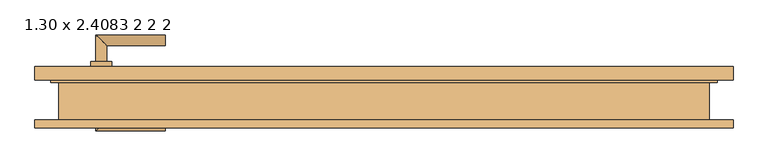
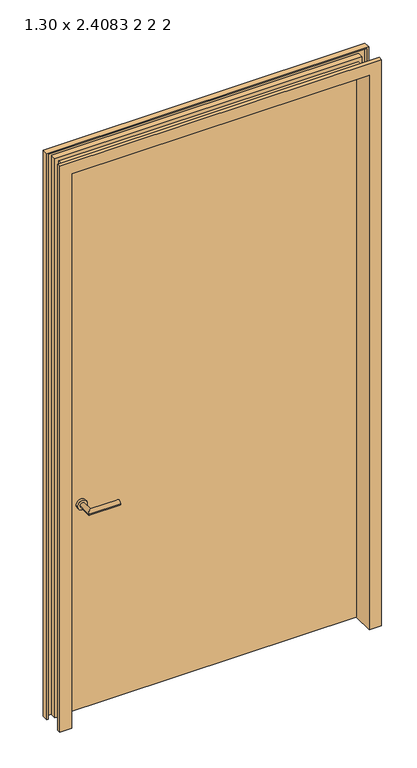
"""IFC4 building model written with IfcOpenShell, lengths in millimetres: door geometry, Drehflügel 1-flg - Stahlzarge : 1.30 x 2.4083 2 2 2."""

from ifc_helpers import new_model, si_unit, point, frame, frame_2d, origin, place, context, project, spatial, polyline, circle_curve, ellipse_curve, trimmed, segment, composite_curve, outline, extrude, faceted_brep, source, transform, mapped, element, save
from ifc_brep_helpers import plane_surface, cylinder_surface, advanced_brep


def door_1_30_x_2_4083_2_2_2_2f50041d(model_context):
    return source(origin(), model_context, "Body", "SolidModel", [
        advanced_brep(
        [(-540.0, 26.9346141, 915.0), (-520.0, 26.9346141, 915.0), (-540.0, -43.0653859, 915.0), (-520.0, -23.0653859, 915.0), (-410.0, -43.0653859, 915.0), (-410.0, -23.0653859, 915.0)],
        [
            (0, 1, circle_curve(frame((-530.0, 26.9346141, 915.0), z_axis=(0.0, 1.0, 0.0), x_axis=(1.0, 0.0, 0.0)), 10.0)),
            (1, 0, circle_curve(frame((-530.0, 26.9346141, 915.0), z_axis=(0.0, 1.0, 0.0), x_axis=(1.0, 0.0, 0.0)), 10.0)),
            (0, 2),
            (2, 3, ellipse_curve(frame((-530.0, -33.0653859, 915.0), z_axis=(-0.7071067811865385, 0.7071067811865565, 0.0), x_axis=(0.7071067811865563, 0.7071067811865386, 0.0)), 14.1421356, 10.0)),
            (3, 1),
            (3, 2, ellipse_curve(frame((-530.0, -33.0653859, 915.0), z_axis=(-0.7071067811865385, 0.7071067811865565, 0.0), x_axis=(0.7071067811865563, 0.7071067811865386, 0.0)), 14.1421356, 10.0)),
            (4, 5, circle_curve(frame((-410.0, -33.0653859, 915.0), z_axis=(1.0, 0.0, 0.0), x_axis=(0.0, 1.0, 0.0)), 10.0)),
            (5, 4, circle_curve(frame((-410.0, -33.0653859, 915.0), z_axis=(1.0, 0.0, 0.0), x_axis=(0.0, 1.0, 0.0)), 10.0)),
            (2, 4),
            (5, 3),
        ],
        [
            plane_surface(frame((-530.0, 26.9346141, -372.7526403), z_axis=(0.0, 1.0, 0.0), x_axis=(0.0, 0.0, 1.0))),
            cylinder_surface(frame((-530.0, 26.9346141, 915.0), z_axis=(0.0, 1.0, 0.0), x_axis=(1.0, 0.0, 0.0)), 10.0),
            plane_surface(frame((-410.0, -33.0653859, -372.7526403), z_axis=(1.0, 0.0, 0.0), x_axis=(0.0, 0.0, 1.0))),
            cylinder_surface(frame((-530.0, -33.0653859, 915.0), z_axis=(-1.0, 0.0, 0.0), x_axis=(0.0, 1.0, 0.0)), 10.0),
        ],
        [
            (0, [[1, 2]]),
            (1, [[-1, 3, 4, 5]]),
            (1, [[-2, -5, 6, -3]]),
            (2, [[7, 8]]),
            (3, [[-4, 9, -8, 10]]),
            (3, [[-6, -10, -7, -9]]),
        ],
    ),
        advanced_brep(
        [(-520.0, 86.9346141, 915.0), (-540.0, 86.9346141, 915.0), (-520.0, 116.9346141, 915.0), (-540.0, 136.9346141, 915.0), (-410.0, 116.9346141, 915.0), (-410.0, 136.9346141, 915.0)],
        [
            (0, 1, circle_curve(frame((-530.0, 86.9346141, 915.0), z_axis=(0.0, -1.0, 0.0), x_axis=(-1.0, 0.0, 0.0)), 10.0)),
            (1, 0, circle_curve(frame((-530.0, 86.9346141, 915.0), z_axis=(0.0, -1.0, 0.0), x_axis=(-1.0, 0.0, 0.0)), 10.0)),
            (0, 2),
            (2, 3, ellipse_curve(frame((-530.0, 126.9346141, 915.0), z_axis=(-0.7071067811865475, -0.7071067811865475, 0.0), x_axis=(0.7071067811865474, -0.7071067811865476, 0.0)), 14.1421356, 10.0)),
            (3, 1),
            (3, 2, ellipse_curve(frame((-530.0, 126.9346141, 915.0), z_axis=(-0.7071067811865475, -0.7071067811865475, 0.0), x_axis=(0.7071067811865474, -0.7071067811865476, 0.0)), 14.1421356, 10.0)),
            (4, 5, circle_curve(frame((-410.0, 126.9346141, 915.0), z_axis=(1.0, 0.0, 0.0), x_axis=(0.0, 1.0, 0.0)), 10.0)),
            (5, 4, circle_curve(frame((-410.0, 126.9346141, 915.0), z_axis=(1.0, 0.0, 0.0), x_axis=(0.0, 1.0, 0.0)), 10.0)),
            (2, 4),
            (5, 3),
        ],
        [
            plane_surface(frame((-530.0, 86.9346141, -372.7526403), z_axis=(0.0, -1.0, 0.0), x_axis=(0.0, 0.0, 1.0))),
            cylinder_surface(frame((-530.0, 86.9346141, 915.0), z_axis=(0.0, -1.0, 0.0), x_axis=(-1.0, 0.0, 0.0)), 10.0),
            plane_surface(frame((-410.0, 126.9346141, -372.7526403), z_axis=(1.0, 0.0, 0.0), x_axis=(0.0, 0.0, 1.0))),
            cylinder_surface(frame((-530.0, 126.9346141, 915.0), z_axis=(-1.0, 0.0, 0.0), x_axis=(0.0, 1.0, 0.0)), 10.0),
        ],
        [
            (0, [[1, 2]]),
            (1, [[-1, 3, 4, 5]]),
            (1, [[-2, -5, 6, -3]]),
            (2, [[7, 8]]),
            (3, [[-4, 9, -8, 10]]),
            (3, [[-6, -10, -7, -9]]),
        ],
    ),
        extrude(outline(composite_curve([segment(trimmed(circle_curve(frame_2d((915.0, -530.0)), 20.0), [point((915.0, -550.0))], [point((915.0, -510.0))], False, "CARTESIAN"), True, "CONTINUOUS"), segment(trimmed(circle_curve(frame_2d((915.0, -530.0)), 20.0), [point((915.0, -510.0))], [point((915.0, -550.0))], False, "CARTESIAN"), True, "CONTINUOUS")], self_intersect=False)), frame((0.0, 16.9346141, 0.0), z_axis=(0.0, 1.0, 0.0), x_axis=(0.0, 0.0, 1.0)), (0.0, 0.0, 1.0), 10.0),
        extrude(outline(composite_curve([segment(trimmed(circle_curve(frame_2d((915.0, -530.0)), 20.0), [point((915.0, -550.0))], [point((915.0, -510.0))], False, "CARTESIAN"), True, "CONTINUOUS"), segment(trimmed(circle_curve(frame_2d((915.0, -530.0)), 20.0), [point((915.0, -510.0))], [point((915.0, -550.0))], False, "CARTESIAN"), True, "CONTINUOUS")], self_intersect=False)), frame((0.0, 76.9346141, 0.0), z_axis=(0.0, 1.0, 0.0), x_axis=(0.0, 0.0, 1.0)), (0.0, 0.0, 1.0), 10.0),
        extrude(outline(polyline([(620.0, 51.9346141), (-620.0, 51.9346141), (-620.0, 76.9346141), (620.0, 76.9346141), (620.0, 51.9346141)])), frame((0.0, 0.0, 15.0), z_axis=(0.0, 0.0, 1.0), x_axis=(1.0, 0.0, 0.0)), (0.0, 0.0, 1.0), 2398.3),
        faceted_brep([(654.4603207, -38.0653859, 15.0), (605.0, -38.0653859, 15.0), (605.0, 51.9346141, 15.0), (620.0, 51.9346141, 15.0), (620.0, 76.9346141, 15.0), (654.4603207, 76.9346141, 15.0), (654.4603207, 51.9346141, 15.0), (649.4603207, 51.9346141, 15.0), (649.4603207, 71.9346141, 15.0), (625.0, 71.9346141, 15.0), (625.0, 46.9346141, 15.0), (610.0, 46.9346141, 15.0), (610.0, -33.0653859, 15.0), (649.4603207, -33.0653859, 15.0), (649.4603207, -23.0653859, 15.0), (654.4603207, -23.0653859, 15.0), (654.4603207, -38.0653859, 2447.7603207), (-654.4603207, -38.0653859, 2447.7603207), (-654.4603207, -38.0653859, 15.0), (-605.0, -38.0653859, 15.0), (-605.0, -38.0653859, 2398.3), (605.0, -38.0653859, 2398.3), (605.0, 51.9346141, 2398.3), (-605.0, 51.9346141, 2398.3), (-605.0, 51.9346141, 15.0), (-620.0, 51.9346141, 15.0), (-620.0, 51.9346141, 2413.3), (620.0, 51.9346141, 2413.3), (620.0, 76.9346141, 2413.3), (-620.0, 76.9346141, 2413.3), (-620.0, 76.9346141, 15.0), (-654.4603207, 76.9346141, 15.0), (-654.4603207, 76.9346141, 2447.7603207), (654.4603207, 76.9346141, 2447.7603207), (654.4603207, 51.9346141, 2447.7603207), (-654.4603207, 51.9346141, 2447.7603207), (-654.4603207, 51.9346141, 15.0), (-649.4603207, 51.9346141, 15.0), (-649.4603207, 51.9346141, 2442.7603207), (649.4603207, 51.9346141, 2442.7603207), (649.4603207, 71.9346141, 2442.7603207), (-649.4603207, 71.9346141, 2442.7603207), (-649.4603207, 71.9346141, 15.0), (-625.0, 71.9346141, 15.0), (-625.0, 71.9346141, 2418.3), (625.0, 71.9346141, 2418.3), (625.0, 46.9346141, 2418.3), (-625.0, 46.9346141, 2418.3), (-625.0, 46.9346141, 15.0), (-610.0, 46.9346141, 15.0), (-610.0, 46.9346141, 2403.3), (610.0, 46.9346141, 2403.3), (610.0, -33.0653859, 2403.3), (-610.0, -33.0653859, 2403.3), (-610.0, -33.0653859, 15.0), (-649.4603207, -33.0653859, 15.0), (-649.4603207, -33.0653859, 2442.7603207), (649.4603207, -33.0653859, 2442.7603207), (649.4603207, -23.0653859, 2442.7603207), (-649.4603207, -23.0653859, 2442.7603207), (-649.4603207, -23.0653859, 15.0), (-654.4603207, -23.0653859, 15.0), (-654.4603207, -23.0653859, 2447.7603207), (654.4603207, -23.0653859, 2447.7603207)], [[[0, 1, 2, 3, 4, 5, 6, 7, 8, 9, 10, 11, 12, 13, 14, 15]], [[1, 0, 16, 17, 18, 19, 20, 21]], [[2, 1, 21, 22]], [[3, 2, 22, 23, 24, 25, 26, 27]], [[4, 3, 27, 28]], [[5, 4, 28, 29, 30, 31, 32, 33]], [[6, 5, 33, 34]], [[7, 6, 34, 35, 36, 37, 38, 39]], [[8, 7, 39, 40]], [[9, 8, 40, 41, 42, 43, 44, 45]], [[10, 9, 45, 46]], [[11, 10, 46, 47, 48, 49, 50, 51]], [[12, 11, 51, 52]], [[13, 12, 52, 53, 54, 55, 56, 57]], [[14, 13, 57, 58]], [[15, 14, 58, 59, 60, 61, 62, 63]], [[0, 15, 63, 16]], [[17, 62, 61, 18]], [[18, 61, 60, 55, 54, 49, 48, 43, 42, 37, 36, 31, 30, 25, 24, 19]], [[23, 20, 19, 24]], [[29, 26, 25, 30]], [[35, 32, 31, 36]], [[41, 38, 37, 42]], [[47, 44, 43, 48]], [[53, 50, 49, 54]], [[59, 56, 55, 60]], [[22, 21, 20, 23]], [[28, 27, 26, 29]], [[34, 33, 32, 35]], [[40, 39, 38, 41]], [[46, 45, 44, 47]], [[52, 51, 50, 53]], [[58, 57, 56, 59]], [[16, 63, 62, 17]]]),
    ])


if __name__ == "__main__":
    model = new_model("IFC4")
    model_context = context("Model", 3, world=origin())
    ifc_project = project(units=[si_unit("LENGTHUNIT", "METRE", prefix="MILLI")], contexts=[model_context])
    site = spatial("IfcSite", under=ifc_project)
    building = spatial("IfcBuilding", under=site)
    placement = place(None, origin())
    door_1_30_x_2_4083_2_2_2_shape = door_1_30_x_2_4083_2_2_2_2f50041d(model_context)
    element("IfcDoor", 1, ObjectType="Drehflügel 1-flg - Stahlzarge : 1.30 x 2.4083 2 2 2", at=placement, inside=building, context=model_context, shape_type="MappedRepresentation", body=[
        mapped(door_1_30_x_2_4083_2_2_2_shape, transform((0.0, 0.0, 0.0), x_axis=(1.0, 0.0, 0.0), y_axis=(0.0, 1.0, 0.0), z_axis=(0.0, 0.0, 1.0))),
    ])
    save(model, "model.ifc")

# Revit data of these elements
# Type "Drehflügel 1-flg - Stahlzarge : 1.30 x 2.4083 2 2 2"
#   Type Mark = "26"
#   Operation = "SingleSwingRight"
#   Keynote = "16.03"
#   Analytic Construction = "Metall"
#   Thermal Resistance (R) = 0.270117 (m²·K)/W
#   Heat Transfer Coefficient (U) = 3.7021 W/(m²·K)
#   Rough Width = 1.260 m
#   Rough Height [instance default] = 2.5083 m
#   Höhe Türgriff [instance default] = 0.900 m
#   Height = 2.4083 m
#   Fußbodenaufbau [instance default] = 0.100 m
#   Width = 1.260 m
#   Sichtbarkeit Sturzlinien [instance default] = yes
#   Türgriff auswählen [instance default] = element 221079
#   Türgriff [instance default] = none
#   Türflügel [instance default] = none
#   Rahmen/Pfosten [instance default] = Metall - Lackiert - Grau
#   Visual Light Transmittance = 0
#   Solar Heat Gain Coefficient = 0
#   Function = (empty or 0)
#   Wall Closure = (empty or 0)
# Element 1 (IfcDoor, "Drehflügel 1-flg - Stahlzarge : 1.30 x 2.4083 2 2 2")
#   Rough Height = 2.4233 m
#   Fußbodenaufbau = 0.015 m
#   Materials on its faces: "Metall - Lackiert - Grau", "Metall - Chrom", "Holz - Birke"
# Materials
#   "Metall - Lackiert - Grau": class "Farbe 1", colour RGB 98 98 98, transparency 0, Cost = 0
#   "Metall - Chrom": class "Metall", colour RGB 247 247 247, transparency 0, Cost = 0
#   "Holz - Birke": class "Holz", colour RGB 213 164 103, transparency 0, Cost = 0
